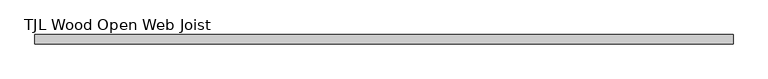
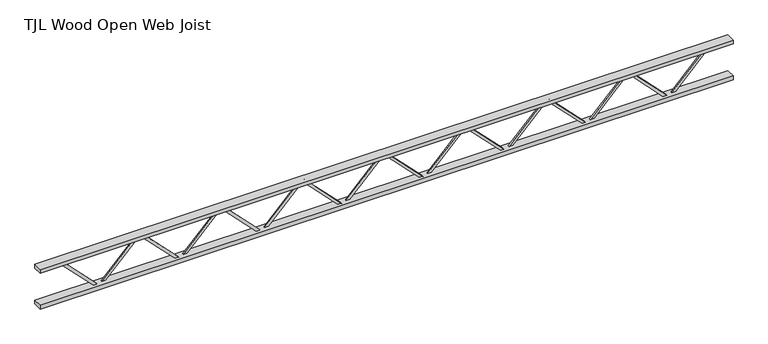
"""IFC4 building model written with IfcOpenShell, lengths in millimetres: beam geometry, TJL Wood Open Web Joist."""

from ifc_helpers import new_model, si_unit, frame, origin, place, context, project, spatial, polyline, outline, extrude, source, transform, mapped, element, save


def tjl_wood_open_web_joist_fdc6c404(model_context):
    return source(origin(), model_context, "Body", "SweptSolid", [
        extrude(outline(polyline([(171.45, 2379.4640625), (196.85, 2379.4640625), (196.85, 2361.4027253), (-171.45, 2002.9253815), (-171.45, 1957.4867188), (-196.85, 1957.4867188), (-196.85, 2013.648056), (171.45, 2372.1253997), (171.45, 2379.4640625)])), frame((0.0, 0.0, 0.0), z_axis=(0.0, 1.0, 0.0), x_axis=(0.0, 0.0, 1.0)), (0.0, 0.0, 1.0), 12.7),
        extrude(outline(polyline([(196.85, 1586.309375), (171.45, 1586.309375), (171.45, 1593.6480378), (-196.85, 1952.1253815), (-196.85, 2008.2867188), (-171.45, 2008.2867188), (-171.45, 1962.848056), (196.85, 1604.3707122), (196.85, 1586.309375)])), frame((0.0, -12.7, 0.0), z_axis=(0.0, 1.0, 0.0), x_axis=(0.0, 0.0, 1.0)), (0.0, 0.0, 1.0), 12.7),
        extrude(outline(polyline([(171.45, 1586.309375), (196.85, 1586.309375), (196.85, 1568.2480378), (-171.45, 1209.770694), (-171.45, 1164.3320313), (-196.85, 1164.3320313), (-196.85, 1220.4933685), (171.45, 1578.9707122), (171.45, 1586.309375)])), frame((0.0, 0.0, 0.0), z_axis=(0.0, 1.0, 0.0), x_axis=(0.0, 0.0, 1.0)), (0.0, 0.0, 1.0), 12.7),
        extrude(outline(polyline([(196.85, 793.1546875), (171.45, 793.1546875), (171.45, 800.4933503), (-196.85, 1158.970694), (-196.85, 1215.1320313), (-171.45, 1215.1320313), (-171.45, 1169.6933685), (196.85, 811.2160247), (196.85, 793.1546875)])), frame((0.0, -12.7, 0.0), z_axis=(0.0, 1.0, 0.0), x_axis=(0.0, 0.0, 1.0)), (0.0, 0.0, 1.0), 12.7),
        extrude(outline(polyline([(171.45, 793.1546875), (196.85, 793.1546875), (196.85, 775.0933503), (-171.45, 416.6160065), (-171.45, 371.1773438), (-196.85, 371.1773438), (-196.85, 427.338681), (171.45, 785.8160247), (171.45, 793.1546875)])), frame((0.0, 0.0, 0.0), z_axis=(0.0, 1.0, 0.0), x_axis=(0.0, 0.0, 1.0)), (0.0, 0.0, 1.0), 12.7),
        extrude(outline(polyline([(196.85, 0.0), (171.45, 0.0), (171.45, 7.3386628), (-196.85, 365.8160065), (-196.85, 421.9773438), (-171.45, 421.9773438), (-171.45, 376.538681), (196.85, 18.0613372), (196.85, 0.0)])), frame((0.0, -12.7, 0.0), z_axis=(0.0, 1.0, 0.0), x_axis=(0.0, 0.0, 1.0)), (0.0, 0.0, 1.0), 12.7),
        extrude(outline(polyline([(171.45, 0.0), (196.85, 0.0), (196.85, -18.0613372), (-171.45, -376.538681), (-171.45, -421.9773437), (-196.85, -421.9773437), (-196.85, -365.8160065), (171.45, -7.3386628), (171.45, 0.0)])), frame((0.0, 0.0, 0.0), z_axis=(0.0, 1.0, 0.0), x_axis=(0.0, 0.0, 1.0)), (0.0, 0.0, 1.0), 12.7),
        extrude(outline(polyline([(196.85, -793.1546875), (171.45, -793.1546875), (171.45, -785.8160247), (-196.85, -427.338681), (-196.85, -371.1773437), (-171.45, -371.1773437), (-171.45, -416.6160065), (196.85, -775.0933503), (196.85, -793.1546875)])), frame((0.0, -12.7, 0.0), z_axis=(0.0, 1.0, 0.0), x_axis=(0.0, 0.0, 1.0)), (0.0, 0.0, 1.0), 12.7),
        extrude(outline(polyline([(171.45, -793.1546875), (196.85, -793.1546875), (196.85, -811.2160247), (-171.45, -1169.6933685), (-171.45, -1215.1320312), (-196.85, -1215.1320312), (-196.85, -1158.970694), (171.45, -800.4933503), (171.45, -793.1546875)])), frame((0.0, 0.0, 0.0), z_axis=(0.0, 1.0, 0.0), x_axis=(0.0, 0.0, 1.0)), (0.0, 0.0, 1.0), 12.7),
        extrude(outline(polyline([(196.85, -1586.309375), (171.45, -1586.309375), (171.45, -1578.9707122), (-196.85, -1220.4933685), (-196.85, -1164.3320312), (-171.45, -1164.3320312), (-171.45, -1209.770694), (196.85, -1568.2480378), (196.85, -1586.309375)])), frame((0.0, -12.7, 0.0), z_axis=(0.0, 1.0, 0.0), x_axis=(0.0, 0.0, 1.0)), (0.0, 0.0, 1.0), 12.7),
        extrude(outline(polyline([(171.45, -1586.309375), (196.85, -1586.309375), (196.85, -1604.3707122), (-171.45, -1962.848056), (-171.45, -2008.2867187), (-196.85, -2008.2867187), (-196.85, -1952.1253815), (171.45, -1593.6480378), (171.45, -1586.309375)])), frame((0.0, 0.0, 0.0), z_axis=(0.0, 1.0, 0.0), x_axis=(0.0, 0.0, 1.0)), (0.0, 0.0, 1.0), 12.7),
        extrude(outline(polyline([(196.85, -2379.4640625), (171.45, -2379.4640625), (171.45, -2372.1253997), (-196.85, -2013.648056), (-196.85, -1957.4867187), (-171.45, -1957.4867187), (-171.45, -2002.9253815), (196.85, -2361.4027253), (196.85, -2379.4640625)])), frame((0.0, -12.7, 0.0), z_axis=(0.0, 1.0, 0.0), x_axis=(0.0, 0.0, 1.0)), (0.0, 0.0, 1.0), 12.7),
        extrude(outline(polyline([(171.45, 3172.61875), (196.85, 3172.61875), (196.85, 3154.5574128), (-171.45, 2796.080069), (-171.45, 2750.6414063), (-196.85, 2750.6414063), (-196.85, 2806.8027435), (171.45, 3165.2800872), (171.45, 3172.61875)])), frame((0.0, 0.0, 0.0), z_axis=(0.0, 1.0, 0.0), x_axis=(0.0, 0.0, 1.0)), (0.0, 0.0, 1.0), 12.7),
        extrude(outline(polyline([(196.85, 2379.4640625), (171.45, 2379.4640625), (171.45, 2386.8027253), (-196.85, 2745.280069), (-196.85, 2801.4414063), (-171.45, 2801.4414063), (-171.45, 2756.0027435), (196.85, 2397.5253997), (196.85, 2379.4640625)])), frame((0.0, -12.7, 0.0), z_axis=(0.0, 1.0, 0.0), x_axis=(0.0, 0.0, 1.0)), (0.0, 0.0, 1.0), 12.7),
        extrude(outline(polyline([(171.45, -2379.4640625), (196.85, -2379.4640625), (196.85, -2397.5253997), (-171.45, -2756.0027435), (-171.45, -2801.4414062), (-196.85, -2801.4414062), (-196.85, -2745.280069), (171.45, -2386.8027253), (171.45, -2379.4640625)])), frame((0.0, 0.0, 0.0), z_axis=(0.0, 1.0, 0.0), x_axis=(0.0, 0.0, 1.0)), (0.0, 0.0, 1.0), 12.7),
        extrude(outline(polyline([(196.85, -3172.61875), (171.45, -3172.61875), (171.45, -3165.2800872), (-196.85, -2806.8027435), (-196.85, -2750.6414062), (-171.45, -2750.6414062), (-171.45, -2796.080069), (196.85, -3154.5574128), (196.85, -3172.61875)])), frame((0.0, -12.7, 0.0), z_axis=(0.0, 1.0, 0.0), x_axis=(0.0, 0.0, 1.0)), (0.0, 0.0, 1.0), 12.7),
        extrude(outline(polyline([(3375.81875, 44.45), (3375.81875, -44.45), (-3375.81875, -44.45), (-3375.81875, 44.45), (3375.81875, 44.45)])), frame((0.0, 0.0, 165.1), z_axis=(0.0, 0.0, 1.0), x_axis=(1.0, 0.0, 0.0)), (0.0, 0.0, 1.0), 38.1),
        extrude(outline(polyline([(3375.81875, 44.45), (3375.81875, -44.45), (-3375.81875, -44.45), (-3375.81875, 44.45), (3375.81875, 44.45)])), frame((0.0, 0.0, -203.2), z_axis=(0.0, 0.0, 1.0), x_axis=(1.0, 0.0, 0.0)), (0.0, 0.0, 1.0), 38.1),
    ])


if __name__ == "__main__":
    model = new_model("IFC4")
    model_context = context("Model", 3, world=origin())
    ifc_project = project(units=[si_unit("LENGTHUNIT", "METRE", prefix="MILLI")], contexts=[model_context])
    site = spatial("IfcSite", under=ifc_project)
    building = spatial("IfcBuilding", under=site)
    placement = place(None, origin())
    tjl_wood_open_web_joist_shape = tjl_wood_open_web_joist_fdc6c404(model_context)
    element("IfcBeam", 1, ObjectType="TJL Wood Open Web Joist : 16\" PREENGINEERED FLOOR TRUSS", at=placement, inside=building, context=model_context, shape_type="MappedRepresentation", body=[
        mapped(tjl_wood_open_web_joist_shape, transform((0.0, 0.0, 0.0), x_axis=(1.0, 0.0, 0.0), y_axis=(0.0, 1.0, 0.0), z_axis=(0.0, 0.0, 1.0))),
    ])
    save(model, "model.ifc")

# Revit data of these elements
# Type "TJL Wood Open Web Joist : 16\" PREENGINEERED FLOOR TRUSS"
#   Web Thickness = 0' - 1"
#   Web Leg = 0' - 1"
#   Start Offset [instance default] = 0' - 0"
#   Top Chord Start Extension [instance default] = 0' - 0"
#   PanelArrayLength [instance default] = 22' - 8"
#   Depth = 1' - 4"
#   PanelWidth [instance default] = 2' - 6.22222"
#   Offset Length 2 [instance default] = 0' - 8"
#   Offset Length 1 [instance default] = 0' - 8"
#   End Panel [instance default] = 0' - 8"
#   End Offset [instance default] = 0' - 0"
#   Top Chord End Extension [instance default] = 0' - 0"
#   Chord Width = 0' - 3 1/2"
#   Chord Depth = 0' - 1 1/2"
#   Bottom Chord Start Extension [instance default] = 0' - 0"
#   Bottom Chord End Extension [instance default] = 0' - 0"
#   Length [instance default] = 24' - 0"
#   PanelArrayNum [instance default] = 9
#   Web Rendering Material = none
#   Structural Material = none
#   Assembly Code = ""
# Element 1 (IfcBeam, "TJL Wood Open Web Joist : 16\" PREENGINEERED FLOOR TRUSS")
#   PanelArrayLength = 20' - 9 13/16"
#   PanelWidth = 2' - 7 29/128"
#   PanelArrayNum = 8
